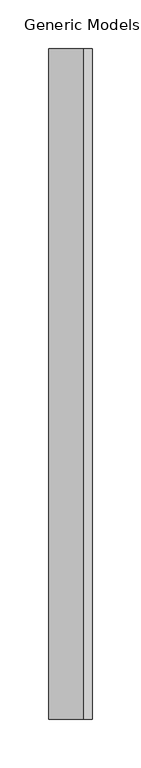
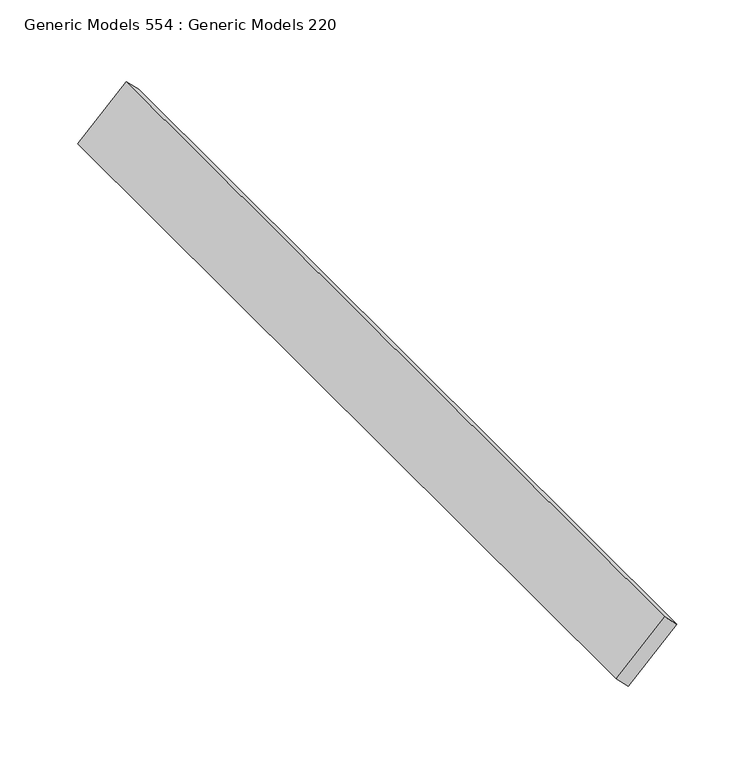
"""IFC4 building model written with IfcOpenShell, lengths in millimetres: proxy geometry, Generic Models 554 : Generic Models 220."""

import ifcopenshell
import ifcopenshell.guid

model = None  # the IFC model being written
_history = None  # IfcOwnerHistory: only IFC2X3 demands one
_inside = {}  # id of a spatial element -> (the spatial element, [elements in it])
_under = {}  # id of a project, library or spatial element -> (it, [spatial elements below it])
_declared = {}  # id of a project -> (the project, [libraries it declares])
_typed = {}  # id of a type object -> (the type object, [elements of that type])
_made_of = {}  # id of a material, layer set ... -> (it, [elements and type objects made of it])


def new_model(schema):
    """Start an empty IFC model of exactly this schema.

    Asked for "IFC4X3", IfcOpenShell would pick the latest addendum, in which some entities
    have other attributes; the version numbers below select the first issue.
    IFC2X3 requires an IfcOwnerHistory on every rooted entity: one is made here for all.
    """
    global model, _history
    if schema == "IFC4X3":
        model = ifcopenshell.file(schema_version=(4, 3, 0, 0))
    else:
        model = ifcopenshell.file(schema=schema)
    _inside.clear()
    _under.clear()
    _declared.clear()
    _typed.clear()
    _made_of.clear()
    _history = None
    if model.schema == "IFC2X3":
        org = make("IfcOrganization", Name="unknown")
        user = make(
            "IfcPersonAndOrganization",
            ThePerson=make("IfcPerson", FamilyName="unknown"),
            TheOrganization=org,
        )
        app = make(
            "IfcApplication",
            ApplicationDeveloper=org,
            Version="unknown",
            ApplicationFullName="unknown",
            ApplicationIdentifier="unknown",
        )
        _history = make(
            "IfcOwnerHistory",
            OwningUser=user,
            OwningApplication=app,
            ChangeAction="ADDED",
            CreationDate=0,
        )
    return model


def make(cls, **values):
    """One entity of the class cls with the attributes given. An attribute that is None is left unset."""
    return model.create_entity(
        cls, **{name: value for name, value in values.items() if value is not None}
    )


def rooted(cls, **values):
    """An entity with a GlobalId (a new one), such as an element, a storey or a relation."""
    return make(cls, GlobalId=ifcopenshell.guid.new(), OwnerHistory=_history, **values)


def si_unit(unit_type, name, prefix=None):
    """IfcSIUnit, for example si_unit("LENGTHUNIT", "METRE", prefix="MILLI")."""
    return make("IfcSIUnit", UnitType=unit_type, Prefix=prefix, Name=name)


def assignment(units):
    """IfcUnitAssignment: the units of a project."""
    return None if units is None else make("IfcUnitAssignment", Units=units)


def point(xyz):
    """IfcCartesianPoint."""
    return None if xyz is None else make("IfcCartesianPoint", Coordinates=xyz)


def direction(xyz):
    """IfcDirection."""
    return None if xyz is None else make("IfcDirection", DirectionRatios=xyz)


def frame(location, z_axis=None, x_axis=None):
    """IfcAxis2Placement3D, a coordinate frame: its origin and axes. An axis left out is left unset."""
    return make(
        "IfcAxis2Placement3D",
        Location=point(location),
        Axis=direction(z_axis),
        RefDirection=direction(x_axis),
    )


def origin():
    """The frame at (0, 0, 0) with its axes left unset."""
    return frame((0.0, 0.0, 0.0))


def place(relative_to, where):
    """IfcLocalPlacement: puts the frame where relative to a parent placement (None: the world)."""
    return make(
        "IfcLocalPlacement", PlacementRelTo=relative_to, RelativePlacement=where
    )


def context(
    kind, dimensions, precision=None, world=None, true_north=None, identifier=None
):
    """IfcGeometricRepresentationContext, for example the 3D "Model" context."""
    return make(
        "IfcGeometricRepresentationContext",
        ContextIdentifier=identifier,
        ContextType=kind,
        CoordinateSpaceDimension=dimensions,
        Precision=precision,
        WorldCoordinateSystem=world,
        TrueNorth=true_north,
    )


def project(units=None, contexts=None):
    """IfcProject with its units and contexts."""
    return rooted(
        "IfcProject",
        Name="project",
        RepresentationContexts=contexts,
        UnitsInContext=assignment(units),
    )


def spatial(cls, under=None, at=None, **own):
    """A site, building, storey or space (cls), placed at a placement, below another one or the project."""
    s = rooted(cls, ObjectPlacement=at, **own)
    if under is not None:
        _under.setdefault(under.id(), (under, []))[1].append(s)
    return s


def polyline(points):
    """IfcPolyline through the points."""
    return make("IfcPolyline", Points=[point(p) for p in points])


def outline(outer, holes=None, kind="AREA"):
    """IfcArbitraryClosedProfileDef: a profile drawn as a closed curve; with holes, ...WithVoids."""
    if holes is None:
        return make("IfcArbitraryClosedProfileDef", ProfileType=kind, OuterCurve=outer)
    return make(
        "IfcArbitraryProfileDefWithVoids",
        ProfileType=kind,
        OuterCurve=outer,
        InnerCurves=holes,
    )


def extrude(swept, where, along, depth):
    """IfcExtrudedAreaSolid: the profile swept, set in the frame where, extruded along a direction by depth."""
    return make(
        "IfcExtrudedAreaSolid",
        SweptArea=swept,
        Position=where,
        ExtrudedDirection=direction(along),
        Depth=depth,
    )


def shape(context_of_items, identifier, shape_type, items):
    """IfcShapeRepresentation: the items that make up one representation, for example the "Body"."""
    return make(
        "IfcShapeRepresentation",
        ContextOfItems=context_of_items,
        RepresentationIdentifier=identifier,
        RepresentationType=shape_type,
        Items=items,
    )


def source(mapping_origin, context_of_items, identifier, shape_type, items):
    """IfcRepresentationMap: a shape defined once, which mapped items show again and again."""
    return make(
        "IfcRepresentationMap",
        MappingOrigin=mapping_origin,
        MappedRepresentation=shape(context_of_items, identifier, shape_type, items),
    )


def transform(
    local_origin,
    x_axis=None,
    y_axis=None,
    z_axis=None,
    scale=None,
    scale2=None,
    scale3=None,
    uniform=True,
):
    """IfcCartesianTransformationOperator3D, or its non-uniform kind. x_axis, y_axis, z_axis: its Axis1, 2, 3."""
    if uniform:
        return make(
            "IfcCartesianTransformationOperator3D",
            Axis1=direction(x_axis),
            Axis2=direction(y_axis),
            LocalOrigin=point(local_origin),
            Scale=scale,
            Axis3=direction(z_axis),
        )
    return make(
        "IfcCartesianTransformationOperator3DnonUniform",
        Axis1=direction(x_axis),
        Axis2=direction(y_axis),
        LocalOrigin=point(local_origin),
        Scale=scale,
        Axis3=direction(z_axis),
        Scale2=scale2,
        Scale3=scale3,
    )


def mapped(mapping_source, mapping_target):
    """IfcMappedItem: shows the shape of a source again, moved by a transform."""
    return make(
        "IfcMappedItem", MappingSource=mapping_source, MappingTarget=mapping_target
    )


def made_of(thing, what):
    """Note that an element or type object is made of a material, layer set ...; save() writes the relation."""
    if what is not None:
        _made_of.setdefault(what.id(), (what, []))[1].append(thing)
    return thing


def element(
    cls,
    number,
    at=None,
    inside=None,
    cuts=None,
    type_object=None,
    material=None,
    context=None,
    identifier="Body",
    shape_type=None,
    held_by="IfcProductDefinitionShape",
    body=None,
    shapes=None,
    **own,
):
    """One element of the class cls, such as IfcWall. Its Tag is "e" and its number.

    at: its placement. inside: the storey or other place that contains it. cuts: it is an
    opening in that element (IfcRelVoidsElement). A single representation is given by context,
    identifier, shape_type and body (its items); several are given by shapes. held_by: the class
    of the entity that holds the representations. save() writes the other relations.
    """
    e = rooted(cls, Tag="e%d" % number, ObjectPlacement=at, **own)
    if body is not None:
        shapes = [shape(context, identifier, shape_type, body)]
    if shapes is not None:
        e.Representation = make(held_by, Representations=shapes)
    if inside is not None:
        _inside.setdefault(inside.id(), (inside, []))[1].append(e)
    if cuts is not None:
        rooted(
            "IfcRelVoidsElement", RelatingBuildingElement=cuts, RelatedOpeningElement=e
        )
    if type_object is not None:
        _typed.setdefault(type_object.id(), (type_object, []))[1].append(e)
    return made_of(e, material)


def aggregate(whole, parts):
    """IfcRelAggregates: a whole, such as a stair, and the parts it consists of."""
    return rooted("IfcRelAggregates", RelatingObject=whole, RelatedObjects=parts)


def save(model, path):
    """Write the relations noted so far, then the file.

    IfcRelAggregates (storeys below a building ...), IfcRelContainedInSpatialStructure (elements
    in a storey), IfcRelDefinesByType, IfcRelAssociatesMaterial and IfcRelDeclares: one each for
    every whole, place, type object, material and project.
    """
    for whole, parts in _under.values():
        aggregate(whole, parts)
    for where, things in _inside.values():
        rooted(
            "IfcRelContainedInSpatialStructure",
            RelatedElements=things,
            RelatingStructure=where,
        )
    for kind, things in _typed.values():
        rooted("IfcRelDefinesByType", RelatedObjects=things, RelatingType=kind)
    for what, things in _made_of.values():
        rooted("IfcRelAssociatesMaterial", RelatedObjects=things, RelatingMaterial=what)
    for by, libraries in _declared.values():
        rooted("IfcRelDeclares", RelatingContext=by, RelatedDefinitions=libraries)
    model.write(path)


def generic_models_554_generic_models_220_e2996ac4(model_context):
    return source(origin(), model_context, "Body", "SweptSolid", [
        extrude(outline(polyline([(0.0, -12.7000001), (0.0, 0.0), (690.8142348, 0.0), (690.8142348, -12.7000001), (0.0, -12.7000001)])), frame((7841.3059863, 4539.4872686, 124557.1399101), z_axis=(0.7071067811868034, 0.0, 0.7071067811862918), x_axis=(0.0, -1.0, 0.0)), (0.0, 0.0, 1.0), 50.8),
    ])


if __name__ == "__main__":
    model = new_model("IFC4")
    model_context = context("Model", 3, world=origin())
    ifc_project = project(units=[si_unit("LENGTHUNIT", "METRE", prefix="MILLI")], contexts=[model_context])
    site = spatial("IfcSite", under=ifc_project)
    building = spatial("IfcBuilding", under=site)
    placement = place(None, origin())
    generic_models_554_generic_models_220_shape = generic_models_554_generic_models_220_e2996ac4(model_context)
    element("IfcBuildingElementProxy", 1, Name="Generic Models 554 : Generic Models 220", ObjectType="Generic Models 554 : Generic Models 220", at=placement, inside=building, context=model_context, shape_type="MappedRepresentation", body=[
        mapped(generic_models_554_generic_models_220_shape, transform((0.0, 0.0, 0.0), x_axis=(1.0, 0.0, 0.0), y_axis=(0.0, 1.0, 0.0), z_axis=(0.0, 0.0, 1.0))),
    ])
    save(model, "model.ifc")

# Revit data of these elements
# Element 1 (IfcBuildingElementProxy, "Generic Models 554 : Generic Models 220")
#   Materials on its faces: "_WOOD TONE ALUMINUM EXTRUSION SLAT BY KNOTWOOD"
# Materials
#   "_WOOD TONE ALUMINUM EXTRUSION SLAT BY KNOTWOOD": class "Generic", colour RGB 177 130 114, transparency 0, Cost = 0
